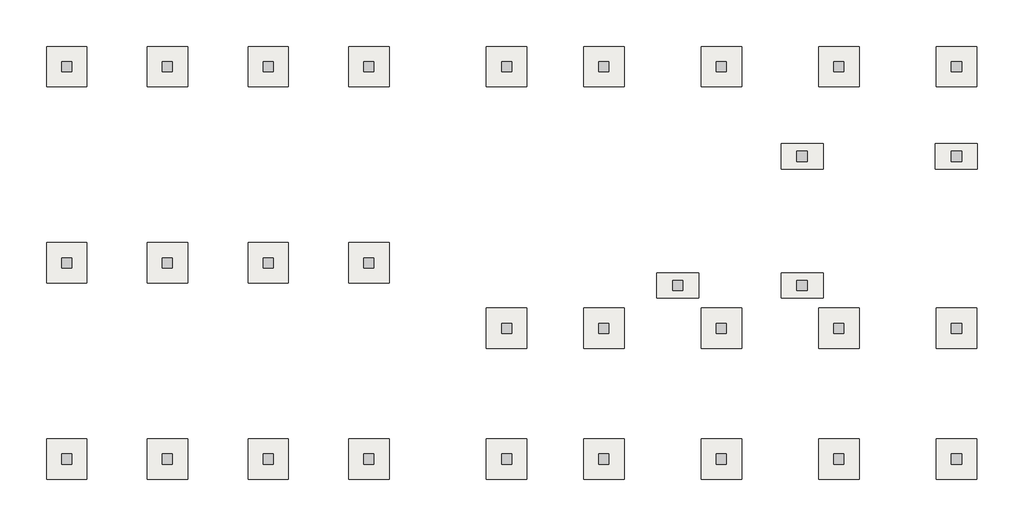
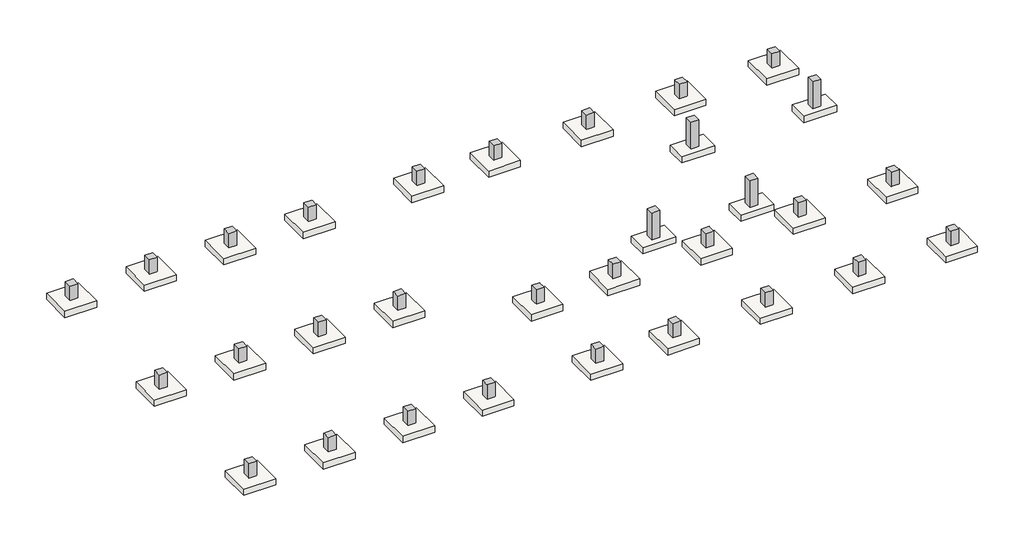
# Not in any storey: 31 columns, 31 slabs.
"""IFC4 building model written with IfcOpenShell, lengths in millimetres."""

import ifcopenshell
import ifcopenshell.guid

model = None  # the IFC model being written
_history = None  # IfcOwnerHistory: only IFC2X3 demands one
_inside = {}  # id of a spatial element -> (the spatial element, [elements in it])
_under = {}  # id of a project, library or spatial element -> (it, [spatial elements below it])
_declared = {}  # id of a project -> (the project, [libraries it declares])
_typed = {}  # id of a type object -> (the type object, [elements of that type])
_made_of = {}  # id of a material, layer set ... -> (it, [elements and type objects made of it])


def new_model(schema):
    """Start an empty IFC model of exactly this schema.

    Asked for "IFC4X3", IfcOpenShell would pick the latest addendum, in which some entities
    have other attributes; the version numbers below select the first issue.
    IFC2X3 requires an IfcOwnerHistory on every rooted entity: one is made here for all.
    """
    global model, _history
    if schema == "IFC4X3":
        model = ifcopenshell.file(schema_version=(4, 3, 0, 0))
    else:
        model = ifcopenshell.file(schema=schema)
    _inside.clear()
    _under.clear()
    _declared.clear()
    _typed.clear()
    _made_of.clear()
    _history = None
    if model.schema == "IFC2X3":
        org = make("IfcOrganization", Name="unknown")
        user = make(
            "IfcPersonAndOrganization",
            ThePerson=make("IfcPerson", FamilyName="unknown"),
            TheOrganization=org,
        )
        app = make(
            "IfcApplication",
            ApplicationDeveloper=org,
            Version="unknown",
            ApplicationFullName="unknown",
            ApplicationIdentifier="unknown",
        )
        _history = make(
            "IfcOwnerHistory",
            OwningUser=user,
            OwningApplication=app,
            ChangeAction="ADDED",
            CreationDate=0,
        )
    return model


def make(cls, **values):
    """One entity of the class cls with the attributes given. An attribute that is None is left unset."""
    return model.create_entity(
        cls, **{name: value for name, value in values.items() if value is not None}
    )


def rooted(cls, **values):
    """An entity with a GlobalId (a new one), such as an element, a storey or a relation."""
    return make(cls, GlobalId=ifcopenshell.guid.new(), OwnerHistory=_history, **values)


def si_unit(unit_type, name, prefix=None):
    """IfcSIUnit, for example si_unit("LENGTHUNIT", "METRE", prefix="MILLI")."""
    return make("IfcSIUnit", UnitType=unit_type, Prefix=prefix, Name=name)


def assignment(units):
    """IfcUnitAssignment: the units of a project."""
    return None if units is None else make("IfcUnitAssignment", Units=units)


def point(xyz):
    """IfcCartesianPoint."""
    return None if xyz is None else make("IfcCartesianPoint", Coordinates=xyz)


def direction(xyz):
    """IfcDirection."""
    return None if xyz is None else make("IfcDirection", DirectionRatios=xyz)


def frame(location, z_axis=None, x_axis=None):
    """IfcAxis2Placement3D, a coordinate frame: its origin and axes. An axis left out is left unset."""
    return make(
        "IfcAxis2Placement3D",
        Location=point(location),
        Axis=direction(z_axis),
        RefDirection=direction(x_axis),
    )


def origin():
    """The frame at (0, 0, 0) with its axes left unset."""
    return frame((0.0, 0.0, 0.0))


def place(relative_to, where):
    """IfcLocalPlacement: puts the frame where relative to a parent placement (None: the world)."""
    return make(
        "IfcLocalPlacement", PlacementRelTo=relative_to, RelativePlacement=where
    )


def context(
    kind, dimensions, precision=None, world=None, true_north=None, identifier=None
):
    """IfcGeometricRepresentationContext, for example the 3D "Model" context."""
    return make(
        "IfcGeometricRepresentationContext",
        ContextIdentifier=identifier,
        ContextType=kind,
        CoordinateSpaceDimension=dimensions,
        Precision=precision,
        WorldCoordinateSystem=world,
        TrueNorth=true_north,
    )


def project(units=None, contexts=None):
    """IfcProject with its units and contexts."""
    return rooted(
        "IfcProject",
        Name="project",
        RepresentationContexts=contexts,
        UnitsInContext=assignment(units),
    )


def spatial(cls, under=None, at=None, **own):
    """A site, building, storey or space (cls), placed at a placement, below another one or the project."""
    s = rooted(cls, ObjectPlacement=at, **own)
    if under is not None:
        _under.setdefault(under.id(), (under, []))[1].append(s)
    return s


def polyline(points):
    """IfcPolyline through the points."""
    return make("IfcPolyline", Points=[point(p) for p in points])


def outline(outer, holes=None, kind="AREA"):
    """IfcArbitraryClosedProfileDef: a profile drawn as a closed curve; with holes, ...WithVoids."""
    if holes is None:
        return make("IfcArbitraryClosedProfileDef", ProfileType=kind, OuterCurve=outer)
    return make(
        "IfcArbitraryProfileDefWithVoids",
        ProfileType=kind,
        OuterCurve=outer,
        InnerCurves=holes,
    )


def extrude(swept, where, along, depth):
    """IfcExtrudedAreaSolid: the profile swept, set in the frame where, extruded along a direction by depth."""
    return make(
        "IfcExtrudedAreaSolid",
        SweptArea=swept,
        Position=where,
        ExtrudedDirection=direction(along),
        Depth=depth,
    )


def faces_of(points, faces, orient=None, outer=None):
    """IfcFace entities. A face is a list of loops; a loop is a list of indices into points, from 0.

    orient and outer hold one flag for each loop. By default every Orientation is true, the
    first loop of a face is its IfcFaceOuterBound and the others are IfcFaceBound.
    """
    made = []
    for i, loops in enumerate(faces):
        bounds = []
        for j, loop in enumerate(loops):
            is_outer = j == 0 if outer is None else outer[i][j]
            bounds.append(
                make(
                    "IfcFaceOuterBound" if is_outer else "IfcFaceBound",
                    Bound=make("IfcPolyLoop", Polygon=[points[k] for k in loop]),
                    Orientation=True if orient is None else orient[i][j],
                )
            )
        made.append(make("IfcFace", Bounds=bounds))
    return made


def faceted_brep(points, faces, orient=None, outer=None, voids=None):
    """IfcFacetedBrep: a solid bounded by flat faces; with voids (closed shells), ...WithVoids."""
    shared = [point(p) for p in points]
    hull = make("IfcClosedShell", CfsFaces=faces_of(shared, faces, orient, outer))
    if voids is None:
        return make("IfcFacetedBrep", Outer=hull)
    return make(
        "IfcFacetedBrepWithVoids",
        Outer=hull,
        Voids=[
            make(cls, CfsFaces=faces_of(shared, fs, o, b)) for cls, fs, o, b in voids
        ],
    )


def shape(context_of_items, identifier, shape_type, items):
    """IfcShapeRepresentation: the items that make up one representation, for example the "Body"."""
    return make(
        "IfcShapeRepresentation",
        ContextOfItems=context_of_items,
        RepresentationIdentifier=identifier,
        RepresentationType=shape_type,
        Items=items,
    )


def source(mapping_origin, context_of_items, identifier, shape_type, items):
    """IfcRepresentationMap: a shape defined once, which mapped items show again and again."""
    return make(
        "IfcRepresentationMap",
        MappingOrigin=mapping_origin,
        MappedRepresentation=shape(context_of_items, identifier, shape_type, items),
    )


def transform(
    local_origin,
    x_axis=None,
    y_axis=None,
    z_axis=None,
    scale=None,
    scale2=None,
    scale3=None,
    uniform=True,
):
    """IfcCartesianTransformationOperator3D, or its non-uniform kind. x_axis, y_axis, z_axis: its Axis1, 2, 3."""
    if uniform:
        return make(
            "IfcCartesianTransformationOperator3D",
            Axis1=direction(x_axis),
            Axis2=direction(y_axis),
            LocalOrigin=point(local_origin),
            Scale=scale,
            Axis3=direction(z_axis),
        )
    return make(
        "IfcCartesianTransformationOperator3DnonUniform",
        Axis1=direction(x_axis),
        Axis2=direction(y_axis),
        LocalOrigin=point(local_origin),
        Scale=scale,
        Axis3=direction(z_axis),
        Scale2=scale2,
        Scale3=scale3,
    )


def mapped(mapping_source, mapping_target):
    """IfcMappedItem: shows the shape of a source again, moved by a transform."""
    return make(
        "IfcMappedItem", MappingSource=mapping_source, MappingTarget=mapping_target
    )


def made_of(thing, what):
    """Note that an element or type object is made of a material, layer set ...; save() writes the relation."""
    if what is not None:
        _made_of.setdefault(what.id(), (what, []))[1].append(thing)
    return thing


def element(
    cls,
    number,
    at=None,
    inside=None,
    cuts=None,
    type_object=None,
    material=None,
    context=None,
    identifier="Body",
    shape_type=None,
    held_by="IfcProductDefinitionShape",
    body=None,
    shapes=None,
    **own,
):
    """One element of the class cls, such as IfcWall. Its Tag is "e" and its number.

    at: its placement. inside: the storey or other place that contains it. cuts: it is an
    opening in that element (IfcRelVoidsElement). A single representation is given by context,
    identifier, shape_type and body (its items); several are given by shapes. held_by: the class
    of the entity that holds the representations. save() writes the other relations.
    """
    e = rooted(cls, Tag="e%d" % number, ObjectPlacement=at, **own)
    if body is not None:
        shapes = [shape(context, identifier, shape_type, body)]
    if shapes is not None:
        e.Representation = make(held_by, Representations=shapes)
    if inside is not None:
        _inside.setdefault(inside.id(), (inside, []))[1].append(e)
    if cuts is not None:
        rooted(
            "IfcRelVoidsElement", RelatingBuildingElement=cuts, RelatedOpeningElement=e
        )
    if type_object is not None:
        _typed.setdefault(type_object.id(), (type_object, []))[1].append(e)
    return made_of(e, material)


def aggregate(whole, parts):
    """IfcRelAggregates: a whole, such as a stair, and the parts it consists of."""
    return rooted("IfcRelAggregates", RelatingObject=whole, RelatedObjects=parts)


def save(model, path):
    """Write the relations noted so far, then the file.

    IfcRelAggregates (storeys below a building ...), IfcRelContainedInSpatialStructure (elements
    in a storey), IfcRelDefinesByType, IfcRelAssociatesMaterial and IfcRelDeclares: one each for
    every whole, place, type object, material and project.
    """
    for whole, parts in _under.values():
        aggregate(whole, parts)
    for where, things in _inside.values():
        rooted(
            "IfcRelContainedInSpatialStructure",
            RelatedElements=things,
            RelatingStructure=where,
        )
    for kind, things in _typed.values():
        rooted("IfcRelDefinesByType", RelatedObjects=things, RelatingType=kind)
    for what, things in _made_of.values():
        rooted("IfcRelAssociatesMaterial", RelatedObjects=things, RelatingMaterial=what)
    for by, libraries in _declared.values():
        rooted("IfcRelDeclares", RelatingContext=by, RelatedDefinitions=libraries)
    model.write(path)


def ft211_footing_rectangular_r1_5fe39465(model_context):
    return source(origin(), model_context, "Body", "SweptSolid", [
        extrude(outline(polyline([(1200.0, 1200.0), (1200.0, -1200.0), (-1200.0, -1200.0), (-1200.0, 1200.0), (1200.0, 1200.0)])), frame((0.0, 0.0, -500.0), z_axis=(0.0, 0.0, 1.0), x_axis=(1.0, 0.0, 0.0)), (0.0, 0.0, 1.0), 500.0),
    ])


def ft211_footing_rectangular_r1_907a7f09(model_context):
    return source(origin(), model_context, "Body", "SweptSolid", [
        extrude(outline(polyline([(1250.0, 750.0), (1250.0, -750.0), (-1250.0, -750.0), (-1250.0, 750.0), (1250.0, 750.0)])), frame((0.0, 0.0, -500.0), z_axis=(0.0, 0.0, 1.0), x_axis=(1.0, 0.0, 0.0)), (0.0, 0.0, 1.0), 500.0),
    ])


model = new_model("IFC4")

# Units and contexts
model_context = context("Model", 3, world=origin())
ifc_project = project(units=[si_unit("LENGTHUNIT", "METRE", prefix="MILLI")], contexts=[model_context])

# Site, building
site = spatial("IfcSite", under=ifc_project)
building = spatial("IfcBuilding", under=site)

# Columns
placement = place(None, origin())
element("IfcColumn", 1, ObjectType="RC_Column_Rectangular : H_SC_ACC_UG PED_W600xL600", at=placement, inside=building, context=model_context, shape_type="Brep", body=[
    faceted_brep([(224.7, 12616.5208589, -1000.0), (224.7, 12016.5208589, -1000.0), (-375.3, 12016.5208589, -1000.0), (-375.3, 12616.5208589, -1000.0), (224.7, 12616.5208589, 150.0), (224.7, 12491.5208589, 150.0), (224.7, 12141.5208589, 150.0), (224.7, 12016.5208589, 150.0), (-375.3, 12016.5208589, 150.0), (-375.3, 12616.5208589, 150.0), (-250.3, 12616.5208589, 150.0), (99.7, 12616.5208589, 150.0)], [[[0, 1, 2, 3]], [[4, 5, 6, 7, 1, 0]], [[7, 8, 2, 1]], [[8, 9, 3, 2]], [[9, 10, 11, 4, 0, 3]], [[4, 11, 10, 9, 8, 7, 6, 5]]]),
])
element("IfcColumn", 2, ObjectType="RC_Column_Rectangular : H_SC_ACC_UG PED_W600xL600", at=placement, inside=building, context=model_context, shape_type="Brep", body=[
    faceted_brep([(6224.7, 12616.5208589, -1000.0), (6224.7, 12016.5208589, -1000.0), (5624.7, 12016.5208589, -1000.0), (5624.7, 12616.5208589, -1000.0), (6224.7, 12616.5208589, 150.0), (6224.7, 12491.5208589, 150.0), (6224.7, 12141.5208589, 150.0), (6224.7, 12016.5208589, 150.0), (5624.7, 12016.5208589, 150.0), (5624.7, 12141.5208589, 150.0), (5624.7, 12491.5208589, 150.0), (5624.7, 12616.5208589, 150.0)], [[[0, 1, 2, 3]], [[4, 5, 6, 7, 1, 0]], [[7, 8, 2, 1]], [[8, 9, 10, 11, 3, 2]], [[11, 4, 0, 3]], [[4, 11, 10, 9, 8, 7, 6, 5]]]),
])
element("IfcColumn", 3, ObjectType="RC_Column_Rectangular : H_SC_ACC_UG PED_W600xL600", at=placement, inside=building, context=model_context, shape_type="Brep", body=[
    faceted_brep([(12224.7, 12616.5208589, -1000.0), (12224.7, 12016.5208589, -1000.0), (11624.7, 12016.5208589, -1000.0), (11624.7, 12616.5208589, -1000.0), (12224.7, 12616.5208589, 150.0), (12224.7, 12491.5208589, 150.0), (12224.7, 12141.5208589, 150.0), (12224.7, 12016.5208589, 150.0), (11624.7, 12016.5208589, 150.0), (11624.7, 12141.5208589, 150.0), (11624.7, 12491.5208589, 150.0), (11624.7, 12616.5208589, 150.0)], [[[0, 1, 2, 3]], [[4, 5, 6, 7, 1, 0]], [[7, 8, 2, 1]], [[8, 9, 10, 11, 3, 2]], [[11, 4, 0, 3]], [[4, 11, 10, 9, 8, 7, 6, 5]]]),
])
element("IfcColumn", 4, ObjectType="RC_Column_Rectangular : H_SC_ACC_UG PED_W600xL600", at=placement, inside=building, context=model_context, shape_type="Brep", body=[
    faceted_brep([(18224.7, 12616.5208589, -1000.0), (18224.7, 12016.5208589, -1000.0), (17624.7, 12016.5208589, -1000.0), (17624.7, 12616.5208589, -1000.0), (18224.7, 12616.5208589, 150.0), (18224.7, 12491.5208589, 150.0), (18224.7, 12141.5208589, 150.0), (18224.7, 12016.5208589, 150.0), (17624.7, 12016.5208589, 150.0), (17624.7, 12141.5208589, 150.0), (17624.7, 12491.5208589, 150.0), (17624.7, 12616.5208589, 150.0)], [[[0, 1, 2, 3]], [[4, 5, 6, 7, 1, 0]], [[7, 8, 2, 1]], [[8, 9, 10, 11, 3, 2]], [[11, 4, 0, 3]], [[4, 11, 10, 9, 8, 7, 6, 5]]]),
])
element("IfcColumn", 5, ObjectType="RC_Column_Rectangular : H_SC_ACC_UG PED_W600xL600", at=placement, inside=building, context=model_context, shape_type="Brep", body=[
    faceted_brep([(224.7, 24316.5208589, -1000.0), (224.7, 23716.5208589, -1000.0), (-375.3, 23716.5208589, -1000.0), (-375.3, 24316.5208589, -1000.0), (224.7, 24316.5208589, 150.0), (224.7, 23716.5208589, 150.0), (99.7, 23716.5208589, 150.0), (-250.3, 23716.5208589, 150.0), (-375.3, 23716.5208589, 150.0), (-375.3, 24316.5208589, 150.0)], [[[0, 1, 2, 3]], [[4, 5, 1, 0]], [[5, 6, 7, 8, 2, 1]], [[8, 9, 3, 2]], [[9, 4, 0, 3]], [[4, 9, 8, 7, 6, 5]]]),
])
element("IfcColumn", 6, ObjectType="RC_Column_Rectangular : H_SC_ACC_UG PED_W600xL600", at=placement, inside=building, context=model_context, shape_type="Brep", body=[
    faceted_brep([(6224.7, 24316.5208589, -1000.0), (6224.7, 23716.5208589, -1000.0), (5624.7, 23716.5208589, -1000.0), (5624.7, 24316.5208589, -1000.0), (6224.7, 24316.5208589, 150.0), (6224.7, 24191.5208589, 150.0), (6224.7, 23841.5208589, 150.0), (6224.7, 23716.5208589, 150.0), (5624.7, 23716.5208589, 150.0), (5624.7, 23841.5208589, 150.0), (5624.7, 24191.5208589, 150.0), (5624.7, 24316.5208589, 150.0)], [[[0, 1, 2, 3]], [[4, 5, 6, 7, 1, 0]], [[7, 8, 2, 1]], [[8, 9, 10, 11, 3, 2]], [[11, 4, 0, 3]], [[4, 11, 10, 9, 8, 7, 6, 5]]]),
])
element("IfcColumn", 7, ObjectType="RC_Column_Rectangular : H_SC_ACC_UG PED_W600xL600", at=placement, inside=building, context=model_context, shape_type="Brep", body=[
    faceted_brep([(12224.7, 24316.5208589, -1000.0), (12224.7, 23716.5208589, -1000.0), (11624.7, 23716.5208589, -1000.0), (11624.7, 24316.5208589, -1000.0), (12224.7, 24316.5208589, 150.0), (12224.7, 24191.5208589, 150.0), (12224.7, 23841.5208589, 150.0), (12224.7, 23716.5208589, 150.0), (11624.7, 23716.5208589, 150.0), (11624.7, 23841.5208589, 150.0), (11624.7, 24191.5208589, 150.0), (11624.7, 24316.5208589, 150.0)], [[[0, 1, 2, 3]], [[4, 5, 6, 7, 1, 0]], [[7, 8, 2, 1]], [[8, 9, 10, 11, 3, 2]], [[11, 4, 0, 3]], [[4, 11, 10, 9, 8, 7, 6, 5]]]),
])
element("IfcColumn", 8, ObjectType="RC_Column_Rectangular : H_SC_ACC_UG PED_W600xL600", at=placement, inside=building, context=model_context, shape_type="Brep", body=[
    faceted_brep([(18224.7, 24316.5208589, -1000.0), (18224.7, 23716.5208589, -1000.0), (17624.7, 23716.5208589, -1000.0), (17624.7, 24316.5208589, -1000.0), (18224.7, 24316.5208589, 150.0), (18224.7, 24191.5208589, 150.0), (18224.7, 23841.5208589, 150.0), (18224.7, 23716.5208589, 150.0), (17624.7, 23716.5208589, 150.0), (17624.7, 23841.5208589, 150.0), (17624.7, 24191.5208589, 150.0), (17624.7, 24316.5208589, 150.0)], [[[0, 1, 2, 3]], [[4, 5, 6, 7, 1, 0]], [[7, 8, 2, 1]], [[8, 9, 10, 11, 3, 2]], [[11, 4, 0, 3]], [[4, 11, 10, 9, 8, 7, 6, 5]]]),
])
element("IfcColumn", 9, ObjectType="RC_Column_Rectangular : H_SC_ACC_UG PED_W600xL600", at=placement, inside=building, context=model_context, shape_type="Brep", body=[
    faceted_brep([(26424.7, 24316.5208589, -1000.0), (26424.7, 23716.5208589, -1000.0), (25824.7, 23716.5208589, -1000.0), (25824.7, 24316.5208589, -1000.0), (26424.7, 24316.5208589, 150.0), (26424.7, 24191.5208589, 150.0), (26424.7, 23841.5208589, 150.0), (26424.7, 23716.5208589, 150.0), (25824.7, 23716.5208589, 150.0), (25824.7, 23841.5208589, 150.0), (25824.7, 24191.5208589, 150.0), (25824.7, 24316.5208589, 150.0)], [[[0, 1, 2, 3]], [[4, 5, 6, 7, 1, 0]], [[7, 8, 2, 1]], [[8, 9, 10, 11, 3, 2]], [[11, 4, 0, 3]], [[4, 11, 10, 9, 8, 7, 6, 5]]]),
])
element("IfcColumn", 10, ObjectType="RC_Column_Rectangular : H_SC_ACC_UG PED_W600xL600", at=placement, inside=building, context=model_context, shape_type="Brep", body=[
    faceted_brep([(32224.7, 24316.5208589, -1000.0), (32224.7, 23716.5208589, -1000.0), (31624.7, 23716.5208589, -1000.0), (31624.7, 24316.5208589, -1000.0), (32224.7, 24316.5208589, 150.0), (32224.7, 24191.5208589, 150.0), (32224.7, 23841.5208589, 150.0), (32224.7, 23716.5208589, 150.0), (31624.7, 23716.5208589, 150.0), (31624.7, 23841.5208589, 150.0), (31624.7, 24191.5208589, 150.0), (31624.7, 24316.5208589, 150.0)], [[[0, 1, 2, 3]], [[4, 5, 6, 7, 1, 0]], [[7, 8, 2, 1]], [[8, 9, 10, 11, 3, 2]], [[11, 4, 0, 3]], [[4, 11, 10, 9, 8, 7, 6, 5]]]),
])
element("IfcColumn", 11, ObjectType="RC_Column_Rectangular : H_SC_ACC_UG PED_W600xL600", at=placement, inside=building, context=model_context, shape_type="Brep", body=[
    faceted_brep([(39224.7, 24316.5208589, -1000.0), (39224.7, 23716.5208589, -1000.0), (38624.7, 23716.5208589, -1000.0), (38624.7, 24316.5208589, -1000.0), (39224.7, 24316.5208589, 150.0), (39224.7, 24191.5208589, 150.0), (39224.7, 23841.5208589, 150.0), (39224.7, 23716.5208589, 150.0), (38624.7, 23716.5208589, 150.0), (38624.7, 23841.5208589, 150.0), (38624.7, 24191.5208589, 150.0), (38624.7, 24316.5208589, 150.0)], [[[0, 1, 2, 3]], [[4, 5, 6, 7, 1, 0]], [[7, 8, 2, 1]], [[8, 9, 10, 11, 3, 2]], [[11, 4, 0, 3]], [[4, 11, 10, 9, 8, 7, 6, 5]]]),
])
element("IfcColumn", 12, ObjectType="RC_Column_Rectangular : H_SC_ACC_UG PED_W600xL600", at=placement, inside=building, context=model_context, shape_type="Brep", body=[
    faceted_brep([(46224.7, 24316.5208589, -1000.0), (46224.7, 23716.5208589, -1000.0), (45624.7, 23716.5208589, -1000.0), (45624.7, 24316.5208589, -1000.0), (46224.7, 24316.5208589, 150.0), (46224.7, 24191.5208589, 150.0), (46224.7, 23841.5208589, 150.0), (46224.7, 23716.5208589, 150.0), (45624.7, 23716.5208589, 150.0), (45624.7, 23841.5208589, 150.0), (45624.7, 24191.5208589, 150.0), (45624.7, 24316.5208589, 150.0)], [[[0, 1, 2, 3]], [[4, 5, 6, 7, 1, 0]], [[7, 8, 2, 1]], [[8, 9, 10, 11, 3, 2]], [[11, 4, 0, 3]], [[4, 11, 10, 9, 8, 7, 6, 5]]]),
])
element("IfcColumn", 13, ObjectType="RC_Column_Rectangular : H_SC_ACC_UG PED_W600xL600", at=placement, inside=building, context=model_context, shape_type="Brep", body=[
    faceted_brep([(53224.7, 24316.5208589, -1000.0), (53224.7, 23716.5208589, -1000.0), (52624.7, 23716.5208589, -1000.0), (52624.7, 24316.5208589, -1000.0), (53224.7, 24316.5208589, 150.0), (53224.7, 23716.5208589, 150.0), (53099.7, 23716.5208589, 150.0), (52749.7, 23716.5208589, 150.0), (52624.7, 23716.5208589, 150.0), (52624.7, 23841.5208589, 150.0), (52624.7, 24191.5208589, 150.0), (52624.7, 24316.5208589, 150.0)], [[[0, 1, 2, 3]], [[4, 5, 1, 0]], [[5, 6, 7, 8, 2, 1]], [[8, 9, 10, 11, 3, 2]], [[11, 4, 0, 3]], [[4, 11, 10, 9, 8, 7, 6, 5]]]),
])
element("IfcColumn", 14, ObjectType="RC_Column_Rectangular : H_SC_ACC_UG PED_W600xL600", at=placement, inside=building, context=model_context, shape_type="Brep", body=[
    faceted_brep([(26424.7, 8716.5208589, -1000.0), (26424.7, 8116.5208589, -1000.0), (25824.7, 8116.5208589, -1000.0), (25824.7, 8716.5208589, -1000.0), (26424.7, 8716.5208589, 150.0), (26424.7, 8591.5208589, 150.0), (26424.7, 8241.5208589, 150.0), (26424.7, 8116.5208589, 150.0), (26299.7, 8116.5208589, 150.0), (25949.7, 8116.5208589, 150.0), (25824.7, 8116.5208589, 150.0), (25824.7, 8241.5208589, 150.0), (25824.7, 8591.5208589, 150.0), (25824.7, 8716.5208589, 150.0)], [[[0, 1, 2, 3]], [[4, 5, 6, 7, 1, 0]], [[7, 8, 9, 10, 2, 1]], [[10, 11, 12, 13, 3, 2]], [[13, 4, 0, 3]], [[4, 13, 12, 11, 10, 9, 8, 7, 6, 5]]]),
])
element("IfcColumn", 15, ObjectType="RC_Column_Rectangular : H_SC_ACC_UG PED_W600xL600", at=placement, inside=building, context=model_context, shape_type="Brep", body=[
    faceted_brep([(32224.7, 8716.5208589, -1000.0), (32224.7, 8116.5208589, -1000.0), (31624.7, 8116.5208589, -1000.0), (31624.7, 8716.5208589, -1000.0), (32224.7, 8716.5208589, 150.0), (32224.7, 8591.5208589, 150.0), (32224.7, 8241.5208589, 150.0), (32224.7, 8116.5208589, 150.0), (31624.7, 8116.5208589, 150.0), (31624.7, 8241.5208589, 150.0), (31624.7, 8591.5208589, 150.0), (31624.7, 8716.5208589, 150.0)], [[[0, 1, 2, 3]], [[4, 5, 6, 7, 1, 0]], [[7, 8, 2, 1]], [[8, 9, 10, 11, 3, 2]], [[11, 4, 0, 3]], [[4, 11, 10, 9, 8, 7, 6, 5]]]),
])
element("IfcColumn", 16, ObjectType="RC_Column_Rectangular : H_SC_ACC_UG PED_W600xL600", at=placement, inside=building, context=model_context, shape_type="Brep", body=[
    faceted_brep([(39224.7, 8716.5208589, -1000.0), (39224.7, 8116.5208589, -1000.0), (38624.7, 8116.5208589, -1000.0), (38624.7, 8716.5208589, -1000.0), (39224.7, 8716.5208589, 150.0), (39224.7, 8591.5208589, 150.0), (39224.7, 8241.5208589, 150.0), (39224.7, 8116.5208589, 150.0), (39099.7, 8116.5208589, 150.0), (38749.7, 8116.5208589, 150.0), (38624.7, 8116.5208589, 150.0), (38624.7, 8241.5208589, 150.0), (38624.7, 8591.5208589, 150.0), (38624.7, 8716.5208589, 150.0)], [[[0, 1, 2, 3]], [[4, 5, 6, 7, 1, 0]], [[7, 8, 9, 10, 2, 1]], [[10, 11, 12, 13, 3, 2]], [[13, 4, 0, 3]], [[4, 13, 12, 11, 10, 9, 8, 7, 6, 5]]]),
])
element("IfcColumn", 17, ObjectType="RC_Column_Rectangular : H_SC_ACC_UG PED_W600xL600", at=placement, inside=building, context=model_context, shape_type="Brep", body=[
    faceted_brep([(46224.7, 8716.5208589, -1000.0), (46224.7, 8116.5208589, -1000.0), (45624.7, 8116.5208589, -1000.0), (45624.7, 8716.5208589, -1000.0), (46224.7, 8716.5208589, 150.0), (46224.7, 8591.5208589, 150.0), (46224.7, 8241.5208589, 150.0), (46224.7, 8116.5208589, 150.0), (46099.7, 8116.5208589, 150.0), (45749.7, 8116.5208589, 150.0), (45624.7, 8116.5208589, 150.0), (45624.7, 8241.5208589, 150.0), (45624.7, 8591.5208589, 150.0), (45624.7, 8716.5208589, 150.0)], [[[0, 1, 2, 3]], [[4, 5, 6, 7, 1, 0]], [[7, 8, 9, 10, 2, 1]], [[10, 11, 12, 13, 3, 2]], [[13, 4, 0, 3]], [[4, 13, 12, 11, 10, 9, 8, 7, 6, 5]]]),
])
element("IfcColumn", 18, ObjectType="RC_Column_Rectangular : H_SC_ACC_UG PED_W600xL600", at=placement, inside=building, context=model_context, shape_type="Brep", body=[
    faceted_brep([(53224.7, 8716.5208589, -1000.0), (53224.7, 8116.5208589, -1000.0), (52624.7, 8116.5208589, -1000.0), (52624.7, 8716.5208589, -1000.0), (53224.7, 8716.5208589, 150.0), (53224.7, 8116.5208589, 150.0), (53099.7, 8116.5208589, 150.0), (52749.7, 8116.5208589, 150.0), (52624.7, 8116.5208589, 150.0), (52624.7, 8241.5208589, 150.0), (52624.7, 8591.5208589, 150.0), (52624.7, 8716.5208589, 150.0), (52749.7, 8716.5208589, 150.0), (53099.7, 8716.5208589, 150.0)], [[[0, 1, 2, 3]], [[4, 5, 1, 0]], [[5, 6, 7, 8, 2, 1]], [[8, 9, 10, 11, 3, 2]], [[11, 12, 13, 4, 0, 3]], [[4, 13, 12, 11, 10, 9, 8, 7, 6, 5]]]),
])
element("IfcColumn", 19, ObjectType="RC_Column_Rectangular : H_SC_ACC_UG PED_W600xL600", at=placement, inside=building, context=model_context, shape_type="Brep", body=[
    faceted_brep([(224.7, 916.5208589, -1000.0), (224.7, 316.5208589, -1000.0), (-375.3, 316.5208589, -1000.0), (-375.3, 916.5208589, -1000.0), (224.7, 916.5208589, 150.0), (224.7, 791.5208589, 150.0), (224.7, 441.5208589, 150.0), (224.7, 316.5208589, 150.0), (-375.3, 316.5208589, 150.0), (-375.3, 916.5208589, 150.0), (-250.3, 916.5208589, 150.0), (99.7, 916.5208589, 150.0)], [[[0, 1, 2, 3]], [[4, 5, 6, 7, 1, 0]], [[7, 8, 2, 1]], [[8, 9, 3, 2]], [[9, 10, 11, 4, 0, 3]], [[4, 11, 10, 9, 8, 7, 6, 5]]]),
])
element("IfcColumn", 20, ObjectType="RC_Column_Rectangular : H_SC_ACC_UG PED_W600xL600", at=placement, inside=building, context=model_context, shape_type="Brep", body=[
    faceted_brep([(6224.7, 916.5208589, -1000.0), (6224.7, 316.5208589, -1000.0), (5624.7, 316.5208589, -1000.0), (5624.7, 916.5208589, -1000.0), (6224.7, 916.5208589, 150.0), (6224.7, 791.5208589, 150.0), (6224.7, 441.5208589, 150.0), (6224.7, 316.5208589, 150.0), (5624.7, 316.5208589, 150.0), (5624.7, 441.5208589, 150.0), (5624.7, 791.5208589, 150.0), (5624.7, 916.5208589, 150.0)], [[[0, 1, 2, 3]], [[4, 5, 6, 7, 1, 0]], [[7, 8, 2, 1]], [[8, 9, 10, 11, 3, 2]], [[11, 4, 0, 3]], [[4, 11, 10, 9, 8, 7, 6, 5]]]),
])
element("IfcColumn", 21, ObjectType="RC_Column_Rectangular : H_SC_ACC_UG PED_W600xL600", at=placement, inside=building, context=model_context, shape_type="Brep", body=[
    faceted_brep([(12224.7, 916.5208589, -1000.0), (12224.7, 316.5208589, -1000.0), (11624.7, 316.5208589, -1000.0), (11624.7, 916.5208589, -1000.0), (12224.7, 916.5208589, 150.0), (12224.7, 791.5208589, 150.0), (12224.7, 441.5208589, 150.0), (12224.7, 316.5208589, 150.0), (11624.7, 316.5208589, 150.0), (11624.7, 441.5208589, 150.0), (11624.7, 791.5208589, 150.0), (11624.7, 916.5208589, 150.0)], [[[0, 1, 2, 3]], [[4, 5, 6, 7, 1, 0]], [[7, 8, 2, 1]], [[8, 9, 10, 11, 3, 2]], [[11, 4, 0, 3]], [[4, 11, 10, 9, 8, 7, 6, 5]]]),
])
element("IfcColumn", 22, ObjectType="RC_Column_Rectangular : H_SC_ACC_UG PED_W600xL600", at=placement, inside=building, context=model_context, shape_type="Brep", body=[
    faceted_brep([(18224.7, 916.5208589, -1000.0), (18224.7, 316.5208589, -1000.0), (17624.7, 316.5208589, -1000.0), (17624.7, 916.5208589, -1000.0), (18224.7, 916.5208589, 150.0), (18224.7, 791.5208589, 150.0), (18224.7, 441.5208589, 150.0), (18224.7, 316.5208589, 150.0), (17624.7, 316.5208589, 150.0), (17624.7, 441.5208589, 150.0), (17624.7, 791.5208589, 150.0), (17624.7, 916.5208589, 150.0)], [[[0, 1, 2, 3]], [[4, 5, 6, 7, 1, 0]], [[7, 8, 2, 1]], [[8, 9, 10, 11, 3, 2]], [[11, 4, 0, 3]], [[4, 11, 10, 9, 8, 7, 6, 5]]]),
])
element("IfcColumn", 23, ObjectType="RC_Column_Rectangular : H_SC_ACC_UG PED_W600xL600", at=placement, inside=building, context=model_context, shape_type="Brep", body=[
    faceted_brep([(26424.7, 916.5208589, -1000.0), (26424.7, 316.5208589, -1000.0), (25824.7, 316.5208589, -1000.0), (25824.7, 916.5208589, -1000.0), (26424.7, 916.5208589, 150.0), (26424.7, 791.5208589, 150.0), (26424.7, 441.5208589, 150.0), (26424.7, 316.5208589, 150.0), (25824.7, 316.5208589, 150.0), (25824.7, 441.5208589, 150.0), (25824.7, 791.5208589, 150.0), (25824.7, 916.5208589, 150.0)], [[[0, 1, 2, 3]], [[4, 5, 6, 7, 1, 0]], [[7, 8, 2, 1]], [[8, 9, 10, 11, 3, 2]], [[11, 4, 0, 3]], [[4, 11, 10, 9, 8, 7, 6, 5]]]),
])
element("IfcColumn", 24, ObjectType="RC_Column_Rectangular : H_SC_ACC_UG PED_W600xL600", at=placement, inside=building, context=model_context, shape_type="Brep", body=[
    faceted_brep([(32224.7, 916.5208589, -1000.0), (32224.7, 316.5208589, -1000.0), (31624.7, 316.5208589, -1000.0), (31624.7, 916.5208589, -1000.0), (32224.7, 916.5208589, 150.0), (32224.7, 791.5208589, 150.0), (32224.7, 441.5208589, 150.0), (32224.7, 316.5208589, 150.0), (31624.7, 316.5208589, 150.0), (31624.7, 441.5208589, 150.0), (31624.7, 791.5208589, 150.0), (31624.7, 916.5208589, 150.0)], [[[0, 1, 2, 3]], [[4, 5, 6, 7, 1, 0]], [[7, 8, 2, 1]], [[8, 9, 10, 11, 3, 2]], [[11, 4, 0, 3]], [[4, 11, 10, 9, 8, 7, 6, 5]]]),
])
element("IfcColumn", 25, ObjectType="RC_Column_Rectangular : H_SC_ACC_UG PED_W600xL600", at=placement, inside=building, context=model_context, shape_type="Brep", body=[
    faceted_brep([(39224.7, 916.5208589, -1000.0), (39224.7, 316.5208589, -1000.0), (38624.7, 316.5208589, -1000.0), (38624.7, 916.5208589, -1000.0), (39224.7, 916.5208589, 150.0), (39224.7, 791.5208589, 150.0), (39224.7, 441.5208589, 150.0), (39224.7, 316.5208589, 150.0), (38624.7, 316.5208589, 150.0), (38624.7, 441.5208589, 150.0), (38624.7, 791.5208589, 150.0), (38624.7, 916.5208589, 150.0)], [[[0, 1, 2, 3]], [[4, 5, 6, 7, 1, 0]], [[7, 8, 2, 1]], [[8, 9, 10, 11, 3, 2]], [[11, 4, 0, 3]], [[4, 11, 10, 9, 8, 7, 6, 5]]]),
])
element("IfcColumn", 26, ObjectType="RC_Column_Rectangular : H_SC_ACC_UG PED_W600xL600", at=placement, inside=building, context=model_context, shape_type="Brep", body=[
    faceted_brep([(46224.7, 916.5208589, -1000.0), (46224.7, 316.5208589, -1000.0), (45624.7, 316.5208589, -1000.0), (45624.7, 916.5208589, -1000.0), (46224.7, 916.5208589, 150.0), (46224.7, 791.5208589, 150.0), (46224.7, 441.5208589, 150.0), (46224.7, 316.5208589, 150.0), (45624.7, 316.5208589, 150.0), (45624.7, 441.5208589, 150.0), (45624.7, 791.5208589, 150.0), (45624.7, 916.5208589, 150.0)], [[[0, 1, 2, 3]], [[4, 5, 6, 7, 1, 0]], [[7, 8, 2, 1]], [[8, 9, 10, 11, 3, 2]], [[11, 4, 0, 3]], [[4, 11, 10, 9, 8, 7, 6, 5]]]),
])
element("IfcColumn", 27, ObjectType="RC_Column_Rectangular : H_SC_ACC_UG PED_W600xL600", at=placement, inside=building, context=model_context, shape_type="Brep", body=[
    faceted_brep([(53224.7, 916.5208589, -1000.0), (53224.7, 316.5208589, -1000.0), (52624.7, 316.5208589, -1000.0), (52624.7, 916.5208589, -1000.0), (53224.7, 916.5208589, 150.0), (53224.7, 316.5208589, 150.0), (52624.7, 316.5208589, 150.0), (52624.7, 441.5208589, 150.0), (52624.7, 791.5208589, 150.0), (52624.7, 916.5208589, 150.0), (52749.7, 916.5208589, 150.0), (53099.7, 916.5208589, 150.0)], [[[0, 1, 2, 3]], [[4, 5, 1, 0]], [[5, 6, 2, 1]], [[6, 7, 8, 9, 3, 2]], [[9, 10, 11, 4, 0, 3]], [[4, 11, 10, 9, 8, 7, 6, 5]]]),
])
element("IfcColumn", 28, ObjectType="RC_Column_Rectangular : H_SC_ACC_UG PED_W600xL600", at=placement, inside=building, context=model_context, shape_type="SweptSolid", body=[
    extrude(outline(polyline([(36624.7, 11266.5208589), (36624.7, 10666.5208589), (36024.7, 10666.5208589), (36024.7, 11266.5208589), (36624.7, 11266.5208589)])), frame((0.0, 0.0, -1000.0), z_axis=(0.0, 0.0, 1.0), x_axis=(1.0, 0.0, 0.0)), (0.0, 0.0, 1.0), 2150.0),
])
element("IfcColumn", 29, ObjectType="RC_Column_Rectangular : H_SC_ACC_UG PED_W600xL600", at=placement, inside=building, context=model_context, shape_type="SweptSolid", body=[
    extrude(outline(polyline([(44024.7, 11266.5208589), (44024.7, 10666.5208589), (43424.7, 10666.5208589), (43424.7, 11266.5208589), (44024.7, 11266.5208589)])), frame((0.0, 0.0, -1000.0), z_axis=(0.0, 0.0, 1.0), x_axis=(1.0, 0.0, 0.0)), (0.0, 0.0, 1.0), 2150.0),
])
element("IfcColumn", 30, ObjectType="RC_Column_Rectangular : H_SC_ACC_UG PED_W600xL600", at=placement, inside=building, context=model_context, shape_type="SweptSolid", body=[
    extrude(outline(polyline([(44024.7, 18966.5208589), (44024.7, 18366.5208589), (43424.7, 18366.5208589), (43424.7, 18966.5208589), (44024.7, 18966.5208589)])), frame((0.0, 0.0, -1000.0), z_axis=(0.0, 0.0, 1.0), x_axis=(1.0, 0.0, 0.0)), (0.0, 0.0, 1.0), 2150.0),
])
element("IfcColumn", 31, ObjectType="RC_Column_Rectangular : H_SC_ACC_UG PED_W600xL600", at=placement, inside=building, context=model_context, shape_type="SweptSolid", body=[
    extrude(outline(polyline([(53224.7, 18966.5208589), (53224.7, 18366.5208589), (52624.7, 18366.5208589), (52624.7, 18966.5208589), (53224.7, 18966.5208589)])), frame((0.0, 0.0, -1000.0), z_axis=(0.0, 0.0, 1.0), x_axis=(1.0, 0.0, 0.0)), (0.0, 0.0, 1.0), 2150.0),
])

# Slabs
element("IfcSlab", 32, ObjectType="FT211-Footing-Rectangular_R1 : H_SF_ACF_W2400xL2400xT500_Bitumen", at=placement, inside=building, context=model_context, shape_type="SweptSolid", body=[
    extrude(outline(polyline([(1124.7, 13516.5208589), (1124.7, 11116.5208589), (-1275.3, 11116.5208589), (-1275.3, 13516.5208589), (1124.7, 13516.5208589)])), frame((0.0, 0.0, -1500.0), z_axis=(0.0, 0.0, 1.0), x_axis=(1.0, 0.0, 0.0)), (0.0, 0.0, 1.0), 500.0),
])
element("IfcSlab", 33, ObjectType="FT211-Footing-Rectangular_R1 : H_SF_ACF_W2400xL2400xT500_Bitumen", at=placement, inside=building, context=model_context, shape_type="SweptSolid", body=[
    extrude(outline(polyline([(7124.7, 13516.5208589), (7124.7, 11116.5208589), (4724.7, 11116.5208589), (4724.7, 13516.5208589), (7124.7, 13516.5208589)])), frame((0.0, 0.0, -1500.0), z_axis=(0.0, 0.0, 1.0), x_axis=(1.0, 0.0, 0.0)), (0.0, 0.0, 1.0), 500.0),
])
element("IfcSlab", 34, ObjectType="FT211-Footing-Rectangular_R1 : H_SF_ACF_W2400xL2400xT500_Bitumen", at=placement, inside=building, context=model_context, shape_type="SweptSolid", body=[
    extrude(outline(polyline([(13124.7, 13516.5208589), (13124.7, 11116.5208589), (10724.7, 11116.5208589), (10724.7, 13516.5208589), (13124.7, 13516.5208589)])), frame((0.0, 0.0, -1500.0), z_axis=(0.0, 0.0, 1.0), x_axis=(1.0, 0.0, 0.0)), (0.0, 0.0, 1.0), 500.0),
])
element("IfcSlab", 35, ObjectType="FT211-Footing-Rectangular_R1 : H_SF_ACF_W2400xL2400xT500_Bitumen", at=placement, inside=building, context=model_context, shape_type="SweptSolid", body=[
    extrude(outline(polyline([(19124.7, 13516.5208589), (19124.7, 11116.5208589), (16724.7, 11116.5208589), (16724.7, 13516.5208589), (19124.7, 13516.5208589)])), frame((0.0, 0.0, -1500.0), z_axis=(0.0, 0.0, 1.0), x_axis=(1.0, 0.0, 0.0)), (0.0, 0.0, 1.0), 500.0),
])
element("IfcSlab", 36, ObjectType="FT211-Footing-Rectangular_R1 : H_SF_ACF_W2400xL2400xT500_Bitumen", at=placement, inside=building, context=model_context, shape_type="SweptSolid", body=[
    extrude(outline(polyline([(27324.7, 9616.5208589), (27324.7, 7216.5208589), (24924.7, 7216.5208589), (24924.7, 9616.5208589), (27324.7, 9616.5208589)])), frame((0.0, 0.0, -1500.0), z_axis=(0.0, 0.0, 1.0), x_axis=(1.0, 0.0, 0.0)), (0.0, 0.0, 1.0), 500.0),
])
element("IfcSlab", 37, ObjectType="FT211-Footing-Rectangular_R1 : H_SF_ACF_W2400xL2400xT500_Bitumen", at=placement, inside=building, context=model_context, shape_type="SweptSolid", body=[
    extrude(outline(polyline([(33124.7, 9616.5208589), (33124.7, 7216.5208589), (30724.7, 7216.5208589), (30724.7, 9616.5208589), (33124.7, 9616.5208589)])), frame((0.0, 0.0, -1500.0), z_axis=(0.0, 0.0, 1.0), x_axis=(1.0, 0.0, 0.0)), (0.0, 0.0, 1.0), 500.0),
])
element("IfcSlab", 38, ObjectType="FT211-Footing-Rectangular_R1 : H_SF_ACF_W2400xL2400xT500_Bitumen", at=placement, inside=building, context=model_context, shape_type="SweptSolid", body=[
    extrude(outline(polyline([(40124.7, 9616.5208589), (40124.7, 7216.5208589), (37724.7, 7216.5208589), (37724.7, 9616.5208589), (40124.7, 9616.5208589)])), frame((0.0, 0.0, -1500.0), z_axis=(0.0, 0.0, 1.0), x_axis=(1.0, 0.0, 0.0)), (0.0, 0.0, 1.0), 500.0),
])
element("IfcSlab", 39, ObjectType="FT211-Footing-Rectangular_R1 : H_SF_ACF_W2400xL2400xT500_Bitumen", at=placement, inside=building, context=model_context, shape_type="SweptSolid", body=[
    extrude(outline(polyline([(47124.7, 9616.5208589), (47124.7, 7216.5208589), (44724.7, 7216.5208589), (44724.7, 9616.5208589), (47124.7, 9616.5208589)])), frame((0.0, 0.0, -1500.0), z_axis=(0.0, 0.0, 1.0), x_axis=(1.0, 0.0, 0.0)), (0.0, 0.0, 1.0), 500.0),
])
element("IfcSlab", 40, ObjectType="FT211-Footing-Rectangular_R1 : H_SF_ACF_W2400xL2400xT500_Bitumen", at=placement, inside=building, context=model_context, shape_type="SweptSolid", body=[
    extrude(outline(polyline([(54124.7, 9616.5208589), (54124.7, 7216.5208589), (51724.7, 7216.5208589), (51724.7, 9616.5208589), (54124.7, 9616.5208589)])), frame((0.0, 0.0, -1500.0), z_axis=(0.0, 0.0, 1.0), x_axis=(1.0, 0.0, 0.0)), (0.0, 0.0, 1.0), 500.0),
])
ft211_footing_rectangular_r1_shape = ft211_footing_rectangular_r1_5fe39465(model_context)
element("IfcSlab", 41, ObjectType="FT211-Footing-Rectangular_R1 : H_SF_ACF_W2400xL2400xT500_Bitumen", at=placement, inside=building, context=model_context, shape_type="MappedRepresentation", body=[
    mapped(ft211_footing_rectangular_r1_shape, transform((-75.3, 24016.5208589, -1000.0), x_axis=(1.0, 0.0, 0.0), y_axis=(0.0, 1.0, 0.0), z_axis=(0.0, 0.0, 1.0))),
])
element("IfcSlab", 42, ObjectType="FT211-Footing-Rectangular_R1 : H_SF_ACF_W2400xL2400xT500_Bitumen", at=placement, inside=building, context=model_context, shape_type="MappedRepresentation", body=[
    mapped(ft211_footing_rectangular_r1_shape, transform((5924.7, 24016.5208589, -1000.0), x_axis=(1.0, 0.0, 0.0), y_axis=(0.0, 1.0, 0.0), z_axis=(0.0, 0.0, 1.0))),
])
element("IfcSlab", 43, ObjectType="FT211-Footing-Rectangular_R1 : H_SF_ACF_W2400xL2400xT500_Bitumen", at=placement, inside=building, context=model_context, shape_type="MappedRepresentation", body=[
    mapped(ft211_footing_rectangular_r1_shape, transform((11924.7, 24016.5208589, -1000.0), x_axis=(1.0, 0.0, 0.0), y_axis=(0.0, 1.0, 0.0), z_axis=(0.0, 0.0, 1.0))),
])
element("IfcSlab", 44, ObjectType="FT211-Footing-Rectangular_R1 : H_SF_ACF_W2400xL2400xT500_Bitumen", at=placement, inside=building, context=model_context, shape_type="MappedRepresentation", body=[
    mapped(ft211_footing_rectangular_r1_shape, transform((17924.7, 24016.5208589, -1000.0), x_axis=(1.0, 0.0, 0.0), y_axis=(0.0, 1.0, 0.0), z_axis=(0.0, 0.0, 1.0))),
])
element("IfcSlab", 45, ObjectType="FT211-Footing-Rectangular_R1 : H_SF_ACF_W2400xL2400xT500_Bitumen", at=placement, inside=building, context=model_context, shape_type="MappedRepresentation", body=[
    mapped(ft211_footing_rectangular_r1_shape, transform((26124.7, 24016.5208589, -1000.0), x_axis=(1.0, 0.0, 0.0), y_axis=(0.0, 1.0, 0.0), z_axis=(0.0, 0.0, 1.0))),
])
element("IfcSlab", 46, ObjectType="FT211-Footing-Rectangular_R1 : H_SF_ACF_W2400xL2400xT500_Bitumen", at=placement, inside=building, context=model_context, shape_type="MappedRepresentation", body=[
    mapped(ft211_footing_rectangular_r1_shape, transform((31924.7, 24016.5208589, -1000.0), x_axis=(1.0, 0.0, 0.0), y_axis=(0.0, 1.0, 0.0), z_axis=(0.0, 0.0, 1.0))),
])
element("IfcSlab", 47, ObjectType="FT211-Footing-Rectangular_R1 : H_SF_ACF_W2400xL2400xT500_Bitumen", at=placement, inside=building, context=model_context, shape_type="MappedRepresentation", body=[
    mapped(ft211_footing_rectangular_r1_shape, transform((38924.7, 24016.5208589, -1000.0), x_axis=(1.0, 0.0, 0.0), y_axis=(0.0, 1.0, 0.0), z_axis=(0.0, 0.0, 1.0))),
])
element("IfcSlab", 48, ObjectType="FT211-Footing-Rectangular_R1 : H_SF_ACF_W2400xL2400xT500_Bitumen", at=placement, inside=building, context=model_context, shape_type="MappedRepresentation", body=[
    mapped(ft211_footing_rectangular_r1_shape, transform((45924.7, 24016.5208589, -1000.0), x_axis=(1.0, 0.0, 0.0), y_axis=(0.0, 1.0, 0.0), z_axis=(0.0, 0.0, 1.0))),
])
element("IfcSlab", 49, ObjectType="FT211-Footing-Rectangular_R1 : H_SF_ACF_W2400xL2400xT500_Bitumen", at=placement, inside=building, context=model_context, shape_type="MappedRepresentation", body=[
    mapped(ft211_footing_rectangular_r1_shape, transform((52924.7, 24016.5208589, -1000.0), x_axis=(1.0, 0.0, 0.0), y_axis=(0.0, 1.0, 0.0), z_axis=(0.0, 0.0, 1.0))),
])
element("IfcSlab", 50, ObjectType="FT211-Footing-Rectangular_R1 : H_SF_ACF_W2400xL2400xT500_Bitumen", at=placement, inside=building, context=model_context, shape_type="MappedRepresentation", body=[
    mapped(ft211_footing_rectangular_r1_shape, transform((-75.3, 616.5208589, -1000.0), x_axis=(1.0, 0.0, 0.0), y_axis=(0.0, 1.0, 0.0), z_axis=(0.0, 0.0, 1.0))),
])
element("IfcSlab", 51, ObjectType="FT211-Footing-Rectangular_R1 : H_SF_ACF_W2400xL2400xT500_Bitumen", at=placement, inside=building, context=model_context, shape_type="MappedRepresentation", body=[
    mapped(ft211_footing_rectangular_r1_shape, transform((5924.7, 616.5208589, -1000.0), x_axis=(1.0, 0.0, 0.0), y_axis=(0.0, 1.0, 0.0), z_axis=(0.0, 0.0, 1.0))),
])
element("IfcSlab", 52, ObjectType="FT211-Footing-Rectangular_R1 : H_SF_ACF_W2400xL2400xT500_Bitumen", at=placement, inside=building, context=model_context, shape_type="MappedRepresentation", body=[
    mapped(ft211_footing_rectangular_r1_shape, transform((11924.7, 616.5208589, -1000.0), x_axis=(1.0, 0.0, 0.0), y_axis=(0.0, 1.0, 0.0), z_axis=(0.0, 0.0, 1.0))),
])
element("IfcSlab", 53, ObjectType="FT211-Footing-Rectangular_R1 : H_SF_ACF_W2400xL2400xT500_Bitumen", at=placement, inside=building, context=model_context, shape_type="MappedRepresentation", body=[
    mapped(ft211_footing_rectangular_r1_shape, transform((17924.7, 616.5208589, -1000.0), x_axis=(1.0, 0.0, 0.0), y_axis=(0.0, 1.0, 0.0), z_axis=(0.0, 0.0, 1.0))),
])
element("IfcSlab", 54, ObjectType="FT211-Footing-Rectangular_R1 : H_SF_ACF_W2400xL2400xT500_Bitumen", at=placement, inside=building, context=model_context, shape_type="MappedRepresentation", body=[
    mapped(ft211_footing_rectangular_r1_shape, transform((26124.7, 616.5208589, -1000.0), x_axis=(1.0, 0.0, 0.0), y_axis=(0.0, 1.0, 0.0), z_axis=(0.0, 0.0, 1.0))),
])
element("IfcSlab", 55, ObjectType="FT211-Footing-Rectangular_R1 : H_SF_ACF_W2400xL2400xT500_Bitumen", at=placement, inside=building, context=model_context, shape_type="MappedRepresentation", body=[
    mapped(ft211_footing_rectangular_r1_shape, transform((31924.7, 616.5208589, -1000.0), x_axis=(1.0, 0.0, 0.0), y_axis=(0.0, 1.0, 0.0), z_axis=(0.0, 0.0, 1.0))),
])
element("IfcSlab", 56, ObjectType="FT211-Footing-Rectangular_R1 : H_SF_ACF_W2400xL2400xT500_Bitumen", at=placement, inside=building, context=model_context, shape_type="MappedRepresentation", body=[
    mapped(ft211_footing_rectangular_r1_shape, transform((38924.7, 616.5208589, -1000.0), x_axis=(1.0, 0.0, 0.0), y_axis=(0.0, 1.0, 0.0), z_axis=(0.0, 0.0, 1.0))),
])
element("IfcSlab", 57, ObjectType="FT211-Footing-Rectangular_R1 : H_SF_ACF_W2400xL2400xT500_Bitumen", at=placement, inside=building, context=model_context, shape_type="MappedRepresentation", body=[
    mapped(ft211_footing_rectangular_r1_shape, transform((45924.7, 616.5208589, -1000.0), x_axis=(1.0, 0.0, 0.0), y_axis=(0.0, 1.0, 0.0), z_axis=(0.0, 0.0, 1.0))),
])
element("IfcSlab", 58, ObjectType="FT211-Footing-Rectangular_R1 : H_SF_ACF_W2400xL2400xT500_Bitumen", at=placement, inside=building, context=model_context, shape_type="MappedRepresentation", body=[
    mapped(ft211_footing_rectangular_r1_shape, transform((52924.7, 616.5208589, -1000.0), x_axis=(1.0, 0.0, 0.0), y_axis=(0.0, 1.0, 0.0), z_axis=(0.0, 0.0, 1.0))),
])
ft211_footing_rectangular_r1_2_shape = ft211_footing_rectangular_r1_907a7f09(model_context)
element("IfcSlab", 59, ObjectType="FT211-Footing-Rectangular_R1 : H_SF_ACF_W2500xL1500xT500_Bitumen", at=placement, inside=building, context=model_context, shape_type="MappedRepresentation", body=[
    mapped(ft211_footing_rectangular_r1_2_shape, transform((36324.7, 10966.5208589, -1000.0), x_axis=(1.0, 0.0, 0.0), y_axis=(0.0, 1.0, 0.0), z_axis=(0.0, 0.0, 1.0))),
])
element("IfcSlab", 60, ObjectType="FT211-Footing-Rectangular_R1 : H_SF_ACF_W2500xL1500xT500_Bitumen", at=placement, inside=building, context=model_context, shape_type="MappedRepresentation", body=[
    mapped(ft211_footing_rectangular_r1_2_shape, transform((43724.7, 10966.5208589, -1000.0), x_axis=(1.0, 0.0, 0.0), y_axis=(0.0, 1.0, 0.0), z_axis=(0.0, 0.0, 1.0))),
])
element("IfcSlab", 61, ObjectType="FT211-Footing-Rectangular_R1 : H_SF_ACF_W2500xL1500xT500_Bitumen", at=placement, inside=building, context=model_context, shape_type="MappedRepresentation", body=[
    mapped(ft211_footing_rectangular_r1_2_shape, transform((43724.7, 18666.5208589, -1000.0), x_axis=(1.0, 0.0, 0.0), y_axis=(0.0, 1.0, 0.0), z_axis=(0.0, 0.0, 1.0))),
])
element("IfcSlab", 62, ObjectType="FT211-Footing-Rectangular_R1 : H_SF_ACF_W2500xL1500xT500_Bitumen", at=placement, inside=building, context=model_context, shape_type="MappedRepresentation", body=[
    mapped(ft211_footing_rectangular_r1_2_shape, transform((52924.7, 18666.5208589, -1000.0), x_axis=(1.0, 0.0, 0.0), y_axis=(0.0, 1.0, 0.0), z_axis=(0.0, 0.0, 1.0))),
])

save(model, "model.ifc")

# Revit data of these elements
# Type "RC_Column_Rectangular : H_SC_ACC_UG PED_W600xL600"
#   Width = 600.000 mm
#   Length = 600.000 mm
#   hec_material3 [instance default] = none
#   hec_material2 [instance default] = none
#   hec_material1 [instance default] = none
#   Structural Material [instance default] = none
#   Description = (empty or 0)
# Type "FT211-Footing-Rectangular_R1 : H_SF_ACF_W2400xL2400xT500_Bitumen"
#   Top bar = "D25@300"
#   Description = "UG Shallow Foundation"
#   Bottom bar = "D20@300"
#   Width = 2400.000 mm
#   Length = 2400.000 mm
#   Foundation Thickness = 500.000 mm
#   Structural Material [instance default] = none
#   Assembly Code = ""
# Type "FT211-Footing-Rectangular_R1 : H_SF_ACF_W2500xL1500xT500_Bitumen"
#   Top bar = "D25@300"
#   Description = "UG Shallow Foundation"
#   Bottom bar = "D20@300"
#   Width = 2500.000 mm
#   Length = 1500.000 mm
#   Foundation Thickness = 500.000 mm
#   Structural Material [instance default] = none
#   Assembly Code = ""
# Elements 1, 2, 3, 4, 5, 6, 7, 8, 9, 10, 11, 12, 13, 14, 15, 16, 17, 18, 19, 20, 21, 22, 23, 24, 25, 26, 27, 28, 29, 30, 31 (IfcColumn, "RC_Column_Rectangular : H_SC_ACC_UG PED_W600xL600")
#   Comments = ""
#   hec_material3 = none
#   hec_material2 = none
#   hec_material1 = none
#   Structural Material = none
#   Phase Created = New Construction
# Elements 32, 33, 34, 35, 36, 37, 38, 39, 40, 41, 42, 43, 44, 45, 46, 47, 48, 49, 50, 51, 52, 53, 54, 55, 56, 57, 58 (IfcSlab, "FT211-Footing-Rectangular_R1 : H_SF_ACF_W2400xL2400xT500_Bitumen")
#   Comments = ""
#   Structural Material = none
#   Phase Created = New Construction
# Elements 59, 60, 61, 62 (IfcSlab, "FT211-Footing-Rectangular_R1 : H_SF_ACF_W2500xL1500xT500_Bitumen")
#   Comments = ""
#   Structural Material = none
#   Phase Created = New Construction
